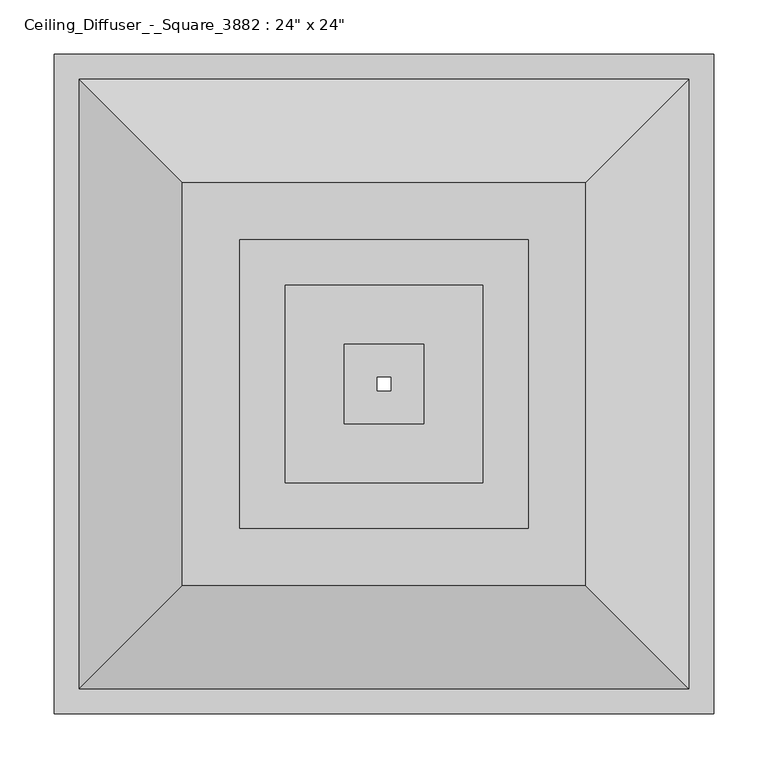
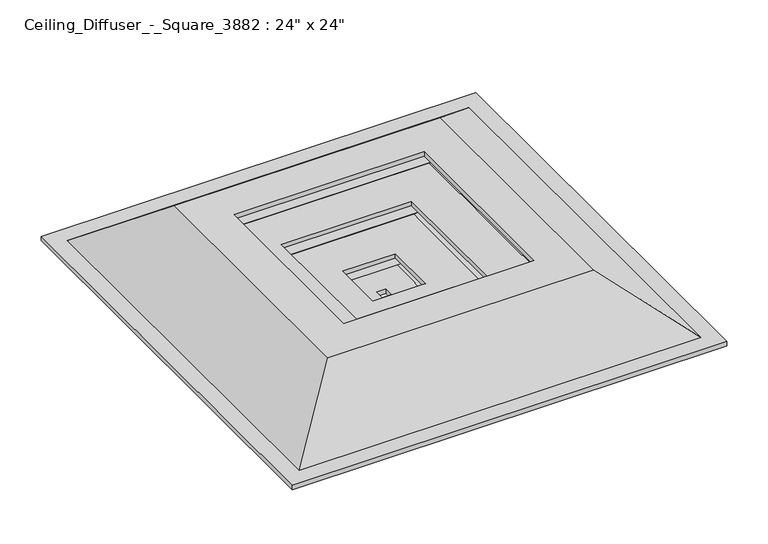
"""IFC4 building model written with IfcOpenShell, lengths in millimetres: proxy geometry."""

import ifcopenshell
import ifcopenshell.guid

model = None  # the IFC model being written
_history = None  # IfcOwnerHistory: only IFC2X3 demands one
_inside = {}  # id of a spatial element -> (the spatial element, [elements in it])
_under = {}  # id of a project, library or spatial element -> (it, [spatial elements below it])
_declared = {}  # id of a project -> (the project, [libraries it declares])
_typed = {}  # id of a type object -> (the type object, [elements of that type])
_made_of = {}  # id of a material, layer set ... -> (it, [elements and type objects made of it])


def new_model(schema):
    """Start an empty IFC model of exactly this schema.

    Asked for "IFC4X3", IfcOpenShell would pick the latest addendum, in which some entities
    have other attributes; the version numbers below select the first issue.
    IFC2X3 requires an IfcOwnerHistory on every rooted entity: one is made here for all.
    """
    global model, _history
    if schema == "IFC4X3":
        model = ifcopenshell.file(schema_version=(4, 3, 0, 0))
    else:
        model = ifcopenshell.file(schema=schema)
    _inside.clear()
    _under.clear()
    _declared.clear()
    _typed.clear()
    _made_of.clear()
    _history = None
    if model.schema == "IFC2X3":
        org = make("IfcOrganization", Name="unknown")
        user = make(
            "IfcPersonAndOrganization",
            ThePerson=make("IfcPerson", FamilyName="unknown"),
            TheOrganization=org,
        )
        app = make(
            "IfcApplication",
            ApplicationDeveloper=org,
            Version="unknown",
            ApplicationFullName="unknown",
            ApplicationIdentifier="unknown",
        )
        _history = make(
            "IfcOwnerHistory",
            OwningUser=user,
            OwningApplication=app,
            ChangeAction="ADDED",
            CreationDate=0,
        )
    return model


def make(cls, **values):
    """One entity of the class cls with the attributes given. An attribute that is None is left unset."""
    return model.create_entity(
        cls, **{name: value for name, value in values.items() if value is not None}
    )


def rooted(cls, **values):
    """An entity with a GlobalId (a new one), such as an element, a storey or a relation."""
    return make(cls, GlobalId=ifcopenshell.guid.new(), OwnerHistory=_history, **values)


def si_unit(unit_type, name, prefix=None):
    """IfcSIUnit, for example si_unit("LENGTHUNIT", "METRE", prefix="MILLI")."""
    return make("IfcSIUnit", UnitType=unit_type, Prefix=prefix, Name=name)


def assignment(units):
    """IfcUnitAssignment: the units of a project."""
    return None if units is None else make("IfcUnitAssignment", Units=units)


def point(xyz):
    """IfcCartesianPoint."""
    return None if xyz is None else make("IfcCartesianPoint", Coordinates=xyz)


def direction(xyz):
    """IfcDirection."""
    return None if xyz is None else make("IfcDirection", DirectionRatios=xyz)


def frame(location, z_axis=None, x_axis=None):
    """IfcAxis2Placement3D, a coordinate frame: its origin and axes. An axis left out is left unset."""
    return make(
        "IfcAxis2Placement3D",
        Location=point(location),
        Axis=direction(z_axis),
        RefDirection=direction(x_axis),
    )


def origin():
    """The frame at (0, 0, 0) with its axes left unset."""
    return frame((0.0, 0.0, 0.0))


def place(relative_to, where):
    """IfcLocalPlacement: puts the frame where relative to a parent placement (None: the world)."""
    return make(
        "IfcLocalPlacement", PlacementRelTo=relative_to, RelativePlacement=where
    )


def context(
    kind, dimensions, precision=None, world=None, true_north=None, identifier=None
):
    """IfcGeometricRepresentationContext, for example the 3D "Model" context."""
    return make(
        "IfcGeometricRepresentationContext",
        ContextIdentifier=identifier,
        ContextType=kind,
        CoordinateSpaceDimension=dimensions,
        Precision=precision,
        WorldCoordinateSystem=world,
        TrueNorth=true_north,
    )


def project(units=None, contexts=None):
    """IfcProject with its units and contexts."""
    return rooted(
        "IfcProject",
        Name="project",
        RepresentationContexts=contexts,
        UnitsInContext=assignment(units),
    )


def spatial(cls, under=None, at=None, **own):
    """A site, building, storey or space (cls), placed at a placement, below another one or the project."""
    s = rooted(cls, ObjectPlacement=at, **own)
    if under is not None:
        _under.setdefault(under.id(), (under, []))[1].append(s)
    return s


def faces_of(points, faces, orient=None, outer=None):
    """IfcFace entities. A face is a list of loops; a loop is a list of indices into points, from 0.

    orient and outer hold one flag for each loop. By default every Orientation is true, the
    first loop of a face is its IfcFaceOuterBound and the others are IfcFaceBound.
    """
    made = []
    for i, loops in enumerate(faces):
        bounds = []
        for j, loop in enumerate(loops):
            is_outer = j == 0 if outer is None else outer[i][j]
            bounds.append(
                make(
                    "IfcFaceOuterBound" if is_outer else "IfcFaceBound",
                    Bound=make("IfcPolyLoop", Polygon=[points[k] for k in loop]),
                    Orientation=True if orient is None else orient[i][j],
                )
            )
        made.append(make("IfcFace", Bounds=bounds))
    return made


def faceted_brep(points, faces, orient=None, outer=None, voids=None):
    """IfcFacetedBrep: a solid bounded by flat faces; with voids (closed shells), ...WithVoids."""
    shared = [point(p) for p in points]
    hull = make("IfcClosedShell", CfsFaces=faces_of(shared, faces, orient, outer))
    if voids is None:
        return make("IfcFacetedBrep", Outer=hull)
    return make(
        "IfcFacetedBrepWithVoids",
        Outer=hull,
        Voids=[
            make(cls, CfsFaces=faces_of(shared, fs, o, b)) for cls, fs, o, b in voids
        ],
    )


def shape(context_of_items, identifier, shape_type, items):
    """IfcShapeRepresentation: the items that make up one representation, for example the "Body"."""
    return make(
        "IfcShapeRepresentation",
        ContextOfItems=context_of_items,
        RepresentationIdentifier=identifier,
        RepresentationType=shape_type,
        Items=items,
    )


def source(mapping_origin, context_of_items, identifier, shape_type, items):
    """IfcRepresentationMap: a shape defined once, which mapped items show again and again."""
    return make(
        "IfcRepresentationMap",
        MappingOrigin=mapping_origin,
        MappedRepresentation=shape(context_of_items, identifier, shape_type, items),
    )


def transform(
    local_origin,
    x_axis=None,
    y_axis=None,
    z_axis=None,
    scale=None,
    scale2=None,
    scale3=None,
    uniform=True,
):
    """IfcCartesianTransformationOperator3D, or its non-uniform kind. x_axis, y_axis, z_axis: its Axis1, 2, 3."""
    if uniform:
        return make(
            "IfcCartesianTransformationOperator3D",
            Axis1=direction(x_axis),
            Axis2=direction(y_axis),
            LocalOrigin=point(local_origin),
            Scale=scale,
            Axis3=direction(z_axis),
        )
    return make(
        "IfcCartesianTransformationOperator3DnonUniform",
        Axis1=direction(x_axis),
        Axis2=direction(y_axis),
        LocalOrigin=point(local_origin),
        Scale=scale,
        Axis3=direction(z_axis),
        Scale2=scale2,
        Scale3=scale3,
    )


def mapped(mapping_source, mapping_target):
    """IfcMappedItem: shows the shape of a source again, moved by a transform."""
    return make(
        "IfcMappedItem", MappingSource=mapping_source, MappingTarget=mapping_target
    )


def made_of(thing, what):
    """Note that an element or type object is made of a material, layer set ...; save() writes the relation."""
    if what is not None:
        _made_of.setdefault(what.id(), (what, []))[1].append(thing)
    return thing


def element(
    cls,
    number,
    at=None,
    inside=None,
    cuts=None,
    type_object=None,
    material=None,
    context=None,
    identifier="Body",
    shape_type=None,
    held_by="IfcProductDefinitionShape",
    body=None,
    shapes=None,
    **own,
):
    """One element of the class cls, such as IfcWall. Its Tag is "e" and its number.

    at: its placement. inside: the storey or other place that contains it. cuts: it is an
    opening in that element (IfcRelVoidsElement). A single representation is given by context,
    identifier, shape_type and body (its items); several are given by shapes. held_by: the class
    of the entity that holds the representations. save() writes the other relations.
    """
    e = rooted(cls, Tag="e%d" % number, ObjectPlacement=at, **own)
    if body is not None:
        shapes = [shape(context, identifier, shape_type, body)]
    if shapes is not None:
        e.Representation = make(held_by, Representations=shapes)
    if inside is not None:
        _inside.setdefault(inside.id(), (inside, []))[1].append(e)
    if cuts is not None:
        rooted(
            "IfcRelVoidsElement", RelatingBuildingElement=cuts, RelatedOpeningElement=e
        )
    if type_object is not None:
        _typed.setdefault(type_object.id(), (type_object, []))[1].append(e)
    return made_of(e, material)


def aggregate(whole, parts):
    """IfcRelAggregates: a whole, such as a stair, and the parts it consists of."""
    return rooted("IfcRelAggregates", RelatingObject=whole, RelatedObjects=parts)


def save(model, path):
    """Write the relations noted so far, then the file.

    IfcRelAggregates (storeys below a building ...), IfcRelContainedInSpatialStructure (elements
    in a storey), IfcRelDefinesByType, IfcRelAssociatesMaterial and IfcRelDeclares: one each for
    every whole, place, type object, material and project.
    """
    for whole, parts in _under.values():
        aggregate(whole, parts)
    for where, things in _inside.values():
        rooted(
            "IfcRelContainedInSpatialStructure",
            RelatedElements=things,
            RelatingStructure=where,
        )
    for kind, things in _typed.values():
        rooted("IfcRelDefinesByType", RelatedObjects=things, RelatingType=kind)
    for what, things in _made_of.values():
        rooted("IfcRelAssociatesMaterial", RelatedObjects=things, RelatingMaterial=what)
    for by, libraries in _declared.values():
        rooted("IfcRelDeclares", RelatingContext=by, RelatedDefinitions=libraries)
    model.write(path)


def proxy_26d92499(model_context):
    return source(origin(), model_context, "Body", "Brep", [
        faceted_brep([(-76.2, -76.2, 2419.35), (-76.2, -76.2, 2413.0), (76.2, -76.2, 2413.0), (76.2, -76.2, 2419.35), (-43.5024597, -43.5024597, 2432.05), (-59.3774597, -59.3774597, 2419.35), (59.3774597, -59.3774597, 2419.35), (43.5024597, -43.5024597, 2432.05), (-6.35, -6.35, 2425.7), (-6.35, -6.35, 2432.05), (6.35, -6.35, 2432.05), (6.35, -6.35, 2425.7), (-57.15, -57.15, 2413.0), (-41.275, -41.275, 2425.7), (41.275, -41.275, 2425.7), (57.15, -57.15, 2413.0), (76.2, 76.2, 2413.0), (76.2, 76.2, 2419.35), (59.3774597, 59.3774597, 2419.35), (43.5024597, 43.5024597, 2432.05), (6.35, 6.35, 2432.05), (6.35, 6.35, 2425.7), (41.275, 41.275, 2425.7), (57.15, 57.15, 2413.0), (-76.2, 76.2, 2413.0), (-76.2, 76.2, 2419.35), (-59.3774597, 59.3774597, 2419.35), (-43.5024597, 43.5024597, 2432.05), (-6.35, 6.35, 2432.05), (-6.35, 6.35, 2425.7), (-41.275, 41.275, 2425.7), (-57.15, 57.15, 2413.0)], [[[0, 1, 2, 3]], [[4, 5, 6, 7]], [[8, 9, 10, 11]], [[12, 13, 14, 15]], [[3, 2, 16, 17]], [[7, 6, 18, 19]], [[11, 10, 20, 21]], [[15, 14, 22, 23]], [[17, 16, 24, 25]], [[19, 18, 26, 27]], [[21, 20, 28, 29]], [[23, 22, 30, 31]], [[25, 24, 1, 0]], [[3, 17, 25, 0], [5, 26, 18, 6]], [[27, 26, 5, 4]], [[7, 19, 27, 4], [9, 28, 20, 10]], [[29, 28, 9, 8]], [[13, 30, 22, 14], [11, 21, 29, 8]], [[31, 30, 13, 12]], [[1, 24, 16, 2], [15, 23, 31, 12]]]),
        faceted_brep([(-152.4, -152.4, 2425.7), (-152.4, -152.4, 2419.35), (152.4, -152.4, 2419.35), (152.4, -152.4, 2425.7), (-98.1644399, -98.1644399, 2455.6304159), (-135.5774597, -135.5774597, 2425.7), (135.5774597, -135.5774597, 2425.7), (98.1644399, -98.1644399, 2455.6304159), (-36.5125, -36.5125, 2449.2804159), (-36.5125, -36.5125, 2455.6304159), (36.5125, -36.5125, 2455.6304159), (36.5125, -36.5125, 2449.2804159), (-133.35, -133.35, 2419.35), (-95.9369802, -95.9369802, 2449.2804159), (95.9369802, -95.9369802, 2449.2804159), (133.35, -133.35, 2419.35), (152.4, 152.4, 2419.35), (152.4, 152.4, 2425.7), (135.5774597, 135.5774597, 2425.7), (98.1644399, 98.1644399, 2455.6304159), (36.5125, 36.5125, 2455.6304159), (36.5125, 36.5125, 2449.2804159), (95.9369802, 95.9369802, 2449.2804159), (133.35, 133.35, 2419.35), (-152.4, 152.4, 2419.35), (-152.4, 152.4, 2425.7), (-135.5774597, 135.5774597, 2425.7), (-98.1644399, 98.1644399, 2455.6304159), (-36.5125, 36.5125, 2455.6304159), (-36.5125, 36.5125, 2449.2804159), (-95.9369802, 95.9369802, 2449.2804159), (-133.35, 133.35, 2419.35)], [[[0, 1, 2, 3]], [[4, 5, 6, 7]], [[8, 9, 10, 11]], [[12, 13, 14, 15]], [[3, 2, 16, 17]], [[7, 6, 18, 19]], [[11, 10, 20, 21]], [[15, 14, 22, 23]], [[17, 16, 24, 25]], [[19, 18, 26, 27]], [[21, 20, 28, 29]], [[23, 22, 30, 31]], [[25, 24, 1, 0]], [[3, 17, 25, 0], [5, 26, 18, 6]], [[27, 26, 5, 4]], [[7, 19, 27, 4], [9, 28, 20, 10]], [[29, 28, 9, 8]], [[13, 30, 22, 14], [11, 21, 29, 8]], [[31, 30, 13, 12]], [[1, 24, 16, 2], [15, 23, 31, 12]]]),
        faceted_brep([(148.3244802, 148.3244802, 2474.6804159), (209.55, 209.55, 2425.7), (209.55, -209.55, 2425.7), (148.3244802, -148.3244802, 2474.6804159), (91.1744802, 91.1744802, 2481.0304159), (91.1744802, 91.1744802, 2474.6804159), (91.1744802, -91.1744802, 2474.6804159), (91.1744802, -91.1744802, 2481.0304159), (211.7774597, 211.7774597, 2432.05), (150.5519399, 150.5519399, 2481.0304159), (150.5519399, -150.5519399, 2481.0304159), (211.7774597, -211.7774597, 2432.05), (228.6, 228.6, 2425.7), (228.6, 228.6, 2432.05), (228.6, -228.6, 2432.05), (228.6, -228.6, 2425.7), (-209.55, -209.55, 2425.7), (-148.3244802, -148.3244802, 2474.6804159), (-91.1744802, -91.1744802, 2474.6804159), (-91.1744802, -91.1744802, 2481.0304159), (-150.5519399, -150.5519399, 2481.0304159), (-211.7774597, -211.7774597, 2432.05), (-228.6, -228.6, 2432.05), (-228.6, -228.6, 2425.7), (-209.55, 209.55, 2425.7), (-148.3244802, 148.3244802, 2474.6804159), (-91.1744802, 91.1744802, 2474.6804159), (-91.1744802, 91.1744802, 2481.0304159), (-150.5519399, 150.5519399, 2481.0304159), (-211.7774597, 211.7774597, 2432.05), (-228.6, 228.6, 2432.05), (-228.6, 228.6, 2425.7)], [[[0, 1, 2, 3]], [[4, 5, 6, 7]], [[8, 9, 10, 11]], [[12, 13, 14, 15]], [[3, 2, 16, 17]], [[7, 6, 18, 19]], [[11, 10, 20, 21]], [[15, 14, 22, 23]], [[17, 16, 24, 25]], [[19, 18, 26, 27]], [[21, 20, 28, 29]], [[23, 22, 30, 31]], [[15, 23, 31, 12], [1, 24, 16, 2]], [[25, 24, 1, 0]], [[3, 17, 25, 0], [5, 26, 18, 6]], [[27, 26, 5, 4]], [[9, 28, 20, 10], [7, 19, 27, 4]], [[29, 28, 9, 8]], [[13, 30, 22, 14], [11, 21, 29, 8]], [[31, 30, 13, 12]]]),
        faceted_brep([(-184.15, 184.15, 2508.25), (-279.4, 279.4, 2432.05), (279.4, 279.4, 2432.05), (184.15, 184.15, 2508.25), (-133.35, 133.35, 2514.6), (-133.35, 133.35, 2508.25), (133.35, 133.35, 2508.25), (133.35, 133.35, 2514.6), (-281.6274597, 281.6274597, 2438.4), (-186.3774597, 186.3774597, 2514.6), (186.3774597, 186.3774597, 2514.6), (281.6274597, 281.6274597, 2438.4), (-304.8, 304.8, 2432.05), (-304.8, 304.8, 2438.4), (304.8, 304.8, 2438.4), (304.8, 304.8, 2432.05), (279.4, -279.4, 2432.05), (184.15, -184.15, 2508.25), (133.35, -133.35, 2508.25), (133.35, -133.35, 2514.6), (186.3774597, -186.3774597, 2514.6), (281.6274597, -281.6274597, 2438.4), (304.8, -304.8, 2438.4), (304.8, -304.8, 2432.05), (-279.4, -279.4, 2432.05), (-184.15, -184.15, 2508.25), (-133.35, -133.35, 2508.25), (-133.35, -133.35, 2514.6), (-186.3774597, -186.3774597, 2514.6), (-281.6274597, -281.6274597, 2438.4), (-304.8, -304.8, 2438.4), (-304.8, -304.8, 2432.05)], [[[0, 1, 2, 3]], [[4, 5, 6, 7]], [[8, 9, 10, 11]], [[12, 13, 14, 15]], [[3, 2, 16, 17]], [[7, 6, 18, 19]], [[11, 10, 20, 21]], [[15, 14, 22, 23]], [[17, 16, 24, 25]], [[19, 18, 26, 27]], [[21, 20, 28, 29]], [[23, 22, 30, 31]], [[15, 23, 31, 12], [1, 24, 16, 2]], [[25, 24, 1, 0]], [[3, 17, 25, 0], [5, 26, 18, 6]], [[27, 26, 5, 4]], [[9, 28, 20, 10], [7, 19, 27, 4]], [[29, 28, 9, 8]], [[13, 30, 22, 14], [11, 21, 29, 8]], [[31, 30, 13, 12]]]),
    ])


if __name__ == "__main__":
    model = new_model("IFC4")
    model_context = context("Model", 3, world=origin())
    ifc_project = project(units=[si_unit("LENGTHUNIT", "METRE", prefix="MILLI")], contexts=[model_context])
    site = spatial("IfcSite", under=ifc_project)
    building = spatial("IfcBuilding", under=site)
    placement = place(None, origin())
    proxy_shape = proxy_26d92499(model_context)
    element("IfcBuildingElementProxy", 1, Name="Ceiling_Diffuser_-_Square_3882 : 24\" x 24\"", ObjectType="Ceiling_Diffuser_-_Square_3882 : 24\" x 24\"", at=placement, inside=building, context=model_context, shape_type="MappedRepresentation", body=[
        mapped(proxy_shape, transform((0.0, 0.0, 0.0), x_axis=(1.0, 0.0, 0.0), y_axis=(0.0, 1.0, 0.0), z_axis=(0.0, 0.0, 1.0))),
    ])
    save(model, "model.ifc")

# Revit data of these elements
# Type "Ceiling_Diffuser_-_Square_3882 : 24\" x 24\""
#   Width = 2' - 0"
#   Length = 2' - 0"
#   Diffuser Finish = none
